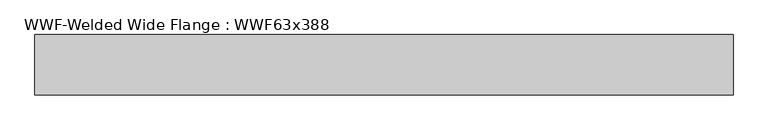
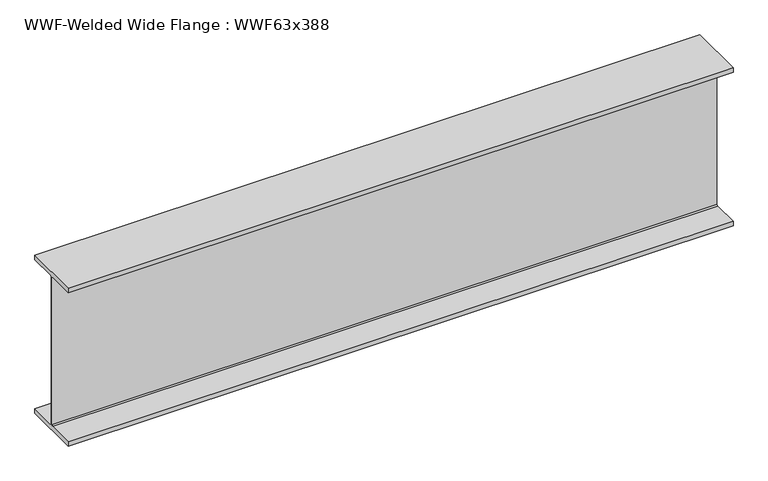
"""IFC4 building model written with IfcOpenShell, lengths in millimetres: beam geometry, WWF-Welded Wide Flange : WWF63x388."""

from ifc_helpers import new_model, si_unit, frame, origin, place, context, project, spatial, polyline, outline, extrude, source, transform, mapped, element, save


def wwf_welded_wide_flange_wwf63x388_644e6ad7(model_context):
    return source(origin(), model_context, "Body", "SweptSolid", [
        extrude(outline(polyline([(274.955, -755.015), (274.955, -799.973), (-274.955, -799.973), (-274.955, -755.015), (-19.05, -755.015), (-8.001, -743.966), (-8.001, 743.966), (-19.05, 755.015), (-274.955, 755.015), (-274.955, 799.973), (274.955, 799.973), (274.955, 755.015), (19.05, 755.015), (8.001, 743.966), (8.001, -743.966), (19.05, -755.015), (274.955, -755.015)])), frame((-3184.5707415, 0.0, 0.0), z_axis=(1.0, 0.0, 0.0), x_axis=(0.0, 1.0, 0.0)), (0.0, 0.0, 1.0), 6369.1344444),
    ])


if __name__ == "__main__":
    model = new_model("IFC4")
    model_context = context("Model", 3, world=origin())
    ifc_project = project(units=[si_unit("LENGTHUNIT", "METRE", prefix="MILLI")], contexts=[model_context])
    site = spatial("IfcSite", under=ifc_project)
    building = spatial("IfcBuilding", under=site)
    placement = place(None, origin())
    wwf_welded_wide_flange_wwf63x388_shape = wwf_welded_wide_flange_wwf63x388_644e6ad7(model_context)
    element("IfcBeam", 1, ObjectType="WWF-Welded Wide Flange : WWF63x388", at=placement, inside=building, context=model_context, shape_type="MappedRepresentation", body=[
        mapped(wwf_welded_wide_flange_wwf63x388_shape, transform((0.0, 0.0, 0.0), x_axis=(1.0, 0.0, 0.0), y_axis=(0.0, 1.0, 0.0), z_axis=(0.0, 0.0, 1.0))),
    ])
    save(model, "model.ifc")

# Revit data of these elements
# Type "WWF-Welded Wide Flange : WWF63x388"
#   Assembly Code = "B10"
#   Nominal d = "12"
#   W = 388
#   Length [instance default] = 1524 mm
#   bf = 549.91 mm
#   d = 1599.946 mm
#   k = 19.05 mm
#   tf = 44.958 mm
#   tw = 16.002 mm
#   A = 0.0735482 m²
#   Structural Material [instance default] = Steel ASTM A572
# Element 1 (IfcBeam, "WWF-Welded Wide Flange : WWF63x388")
#   Structural Material = Metal - Steel 43-275
#   Materials on its faces: "Metal - Steel 43-275"
# Materials
#   "Steel ASTM A572": class "Metal", colour RGB 247 247 247, transparency 0, Description = "Structural steel, high strength low alloy, ASTM - A572 - 50", Cost = 0
#   "Metal - Steel 43-275": class "Metal", colour RGB 247 247 247, transparency 0, Cost = 0
